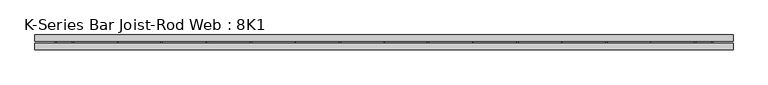
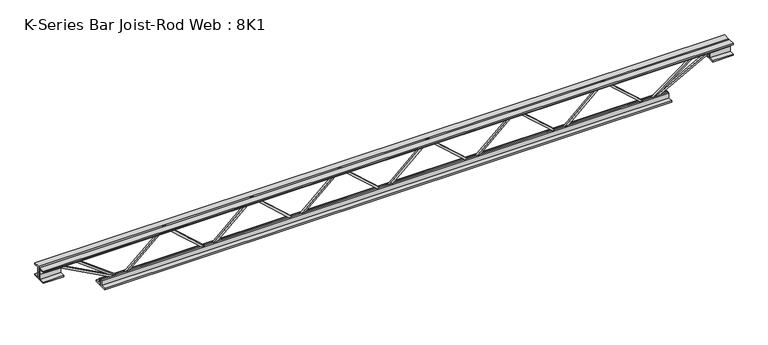
"""IFC4 building model written with IfcOpenShell, lengths in millimetres: beam geometry, K-Series Bar Joist-Rod Web : 8K1."""

from ifc_helpers import new_model, si_unit, frame, origin, place, context, project, spatial, polyline, outline, extrude, source, transform, mapped, element, save


def k_series_bar_joist_rod_web_8k1_279f3ebc(model_context):
    return source(origin(), model_context, "Body", "SweptSolid", [
        extrude(outline(polyline([(-90.4875, 437.278907), (-100.0125, 437.278907), (-100.0125, 442.2774605), (90.4875, 654.566914), (90.4875, 657.269807), (-100.0125, 869.5592605), (-100.0125, 874.557814), (-90.4875, 874.557814), (-90.4875, 873.2063675), (100.0125, 660.916914), (100.0125, 650.919807), (-90.4875, 438.6303535), (-90.4875, 437.278907)])), frame((0.0, -4.7625, 0.0), z_axis=(0.0, 1.0, 0.0), x_axis=(0.0, 0.0, 1.0)), (0.0, 0.0, 1.0), 9.525),
        extrude(outline(polyline([(-90.4875, 0.0), (-100.0125, 0.0), (-100.0125, 4.9985535), (90.4875, 217.288007), (90.4875, 219.9909), (-100.0125, 432.2803535), (-100.0125, 437.278907), (-90.4875, 437.278907), (-90.4875, 435.9274605), (100.0125, 223.638007), (100.0125, 213.6409), (-90.4875, 1.3514465), (-90.4875, 0.0)])), frame((0.0, -4.7625, 0.0), z_axis=(0.0, 1.0, 0.0), x_axis=(0.0, 0.0, 1.0)), (0.0, 0.0, 1.0), 9.525),
        extrude(outline(polyline([(-90.4875, -437.278907), (-100.0125, -437.278907), (-100.0125, -432.2803535), (90.4875, -219.9909), (90.4875, -217.288007), (-100.0125, -4.9985535), (-100.0125, 0.0), (-90.4875, 0.0), (-90.4875, -1.3514465), (100.0125, -213.6409), (100.0125, -223.638007), (-90.4875, -435.9274605), (-90.4875, -437.278907)])), frame((0.0, -4.7625, 0.0), z_axis=(0.0, 1.0, 0.0), x_axis=(0.0, 0.0, 1.0)), (0.0, 0.0, 1.0), 9.525),
        extrude(outline(polyline([(-90.4875, -874.557814), (-100.0125, -874.557814), (-100.0125, -869.5592605), (90.4875, -657.269807), (90.4875, -654.566914), (-100.0125, -442.2774605), (-100.0125, -437.278907), (-90.4875, -437.278907), (-90.4875, -438.6303535), (100.0125, -650.919807), (100.0125, -660.916914), (-90.4875, -873.2063675), (-90.4875, -874.557814)])), frame((0.0, -4.7625, 0.0), z_axis=(0.0, 1.0, 0.0), x_axis=(0.0, 0.0, 1.0)), (0.0, 0.0, 1.0), 9.525),
        extrude(outline(polyline([(-90.4875, 874.557814), (-100.0125, 874.557814), (-100.0125, 879.5563675), (90.4875, 1091.845821), (90.4875, 1094.548714), (-100.0125, 1306.8381675), (-100.0125, 1311.836721), (-90.4875, 1311.836721), (-90.4875, 1310.4852745), (100.0125, 1098.195821), (100.0125, 1088.198714), (-90.4875, 875.9092605), (-90.4875, 874.557814)])), frame((0.0, -4.7625, 0.0), z_axis=(0.0, 1.0, 0.0), x_axis=(0.0, 0.0, 1.0)), (0.0, 0.0, 1.0), 9.525),
        extrude(outline(polyline([(-90.4875, -1311.836721), (-100.0125, -1311.836721), (-100.0125, -1306.8381675), (90.4875, -1094.548714), (90.4875, -1091.845821), (-100.0125, -879.5563675), (-100.0125, -874.557814), (-90.4875, -874.557814), (-90.4875, -875.9092605), (100.0125, -1088.198714), (100.0125, -1098.195821), (-90.4875, -1310.4852745), (-90.4875, -1311.836721)])), frame((0.0, -4.7625, 0.0), z_axis=(0.0, 1.0, 0.0), x_axis=(0.0, 0.0, 1.0)), (0.0, 0.0, 1.0), 9.525),
        extrude(outline(polyline([(4.7625, 101.6), (36.5125, 101.6), (36.5125, 95.25), (11.1125, 95.25), (11.1125, 69.85), (4.7625, 69.85), (4.7625, 101.6)])), frame((-1718.236721, 0.0, 0.0), z_axis=(1.0, 0.0, 0.0), x_axis=(0.0, 1.0, 0.0)), (0.0, 0.0, 1.0), 3436.473442),
        extrude(outline(polyline([(-4.7625, 101.6), (-4.7625, 69.85), (-11.1125, 69.85), (-11.1125, 95.25), (-36.5125, 95.25), (-36.5125, 101.6), (-4.7625, 101.6)])), frame((-1718.236721, 0.0, 0.0), z_axis=(1.0, 0.0, 0.0), x_axis=(0.0, 1.0, 0.0)), (0.0, 0.0, 1.0), 3436.473442),
        extrude(outline(polyline([(-4.7625, 38.1), (-36.5125, 38.1), (-36.5125, 44.45), (-11.1125, 44.45), (-11.1125, 69.85), (-4.7625, 69.85), (-4.7625, 38.1)])), frame((-1718.236721, 0.0, 0.0), z_axis=(1.0, 0.0, 0.0), x_axis=(0.0, 1.0, 0.0)), (0.0, 0.0, 1.0), 101.6),
        extrude(outline(polyline([(36.5125, 38.1), (4.7625, 38.1), (4.7625, 69.85), (11.1125, 69.85), (11.1125, 44.45), (36.5125, 44.45), (36.5125, 38.1)])), frame((-1718.236721, 0.0, 0.0), z_axis=(1.0, 0.0, 0.0), x_axis=(0.0, 1.0, 0.0)), (0.0, 0.0, 1.0), 101.6),
        extrude(outline(polyline([(4.7625, 38.1), (4.7625, 69.85), (11.1125, 69.85), (11.1125, 44.45), (36.5125, 44.45), (36.5125, 38.1), (4.7625, 38.1)])), frame((1616.636721, 0.0, 0.0), z_axis=(1.0, 0.0, 0.0), x_axis=(0.0, 1.0, 0.0)), (0.0, 0.0, 1.0), 101.6),
        extrude(outline(polyline([(-4.7625, 38.1), (-36.5125, 38.1), (-36.5125, 44.45), (-11.1125, 44.45), (-11.1125, 69.85), (-4.7625, 69.85), (-4.7625, 38.1)])), frame((1616.636721, 0.0, 0.0), z_axis=(1.0, 0.0, 0.0), x_axis=(0.0, 1.0, 0.0)), (0.0, 0.0, 1.0), 101.6),
        extrude(outline(polyline([(4.7625, -101.6), (4.7625, -69.85), (11.1125, -69.85), (11.1125, -95.25), (36.5125, -95.25), (36.5125, -101.6), (4.7625, -101.6)])), frame((-1413.436721, 0.0, 0.0), z_axis=(1.0, 0.0, 0.0), x_axis=(0.0, 1.0, 0.0)), (0.0, 0.0, 1.0), 2826.873442),
        extrude(outline(polyline([(-4.7625, -101.6), (-36.5125, -101.6), (-36.5125, -95.25), (-11.1125, -95.25), (-11.1125, -69.85), (-4.7625, -69.85), (-4.7625, -101.6)])), frame((-1413.436721, 0.0, 0.0), z_axis=(1.0, 0.0, 0.0), x_axis=(0.0, 1.0, 0.0)), (0.0, 0.0, 1.0), 2826.873442),
        extrude(outline(polyline([(0.0, -9.525), (0.0, 0.0), (346.6425392, 0.0), (346.6425392, -9.525), (0.0, -9.525)])), frame((-1618.9050195, 4.7625, 65.662372), z_axis=(0.47628314854008014, 0.0, 0.8792919665371384), x_axis=(0.8792919665371384, 0.0, -0.47628314854008014)), (0.0, 0.0, 1.0), 9.525),
        extrude(outline(polyline([(0.0, -9.525), (0.0, 0.0), (273.973029, 0.0), (273.973029, -9.525), (0.0, -9.525)])), frame((-1533.346124, 4.7625, 66.049369), z_axis=(0.6026140623855752, 0.0, 0.7980327636226184), x_axis=(0.7980327636226184, 0.0, -0.6026140623855752)), (0.0, 0.0, 1.0), 9.525),
        extrude(outline(polyline([(0.0, -9.525), (0.0, 0.0), (346.6425392, 0.0), (346.6425392, -9.525), (0.0, -9.525)])), frame((1618.9050195, -4.7625, 65.662372), z_axis=(-0.4762831485400414, 0.0, 0.8792919665371594), x_axis=(-0.8792919665371594, 0.0, -0.4762831485400414)), (0.0, 0.0, 1.0), 9.525),
        extrude(outline(polyline([(0.0, -9.525), (0.0, 0.0), (273.973029, 0.0), (273.973029, -9.525), (0.0, -9.525)])), frame((1533.346124, -4.7625, 66.049369), z_axis=(-0.602614062385554, 0.0, 0.7980327636226345), x_axis=(-0.7980327636226345, 0.0, -0.602614062385554)), (0.0, 0.0, 1.0), 9.525),
    ])


if __name__ == "__main__":
    model = new_model("IFC4")
    model_context = context("Model", 3, world=origin())
    ifc_project = project(units=[si_unit("LENGTHUNIT", "METRE", prefix="MILLI")], contexts=[model_context])
    site = spatial("IfcSite", under=ifc_project)
    building = spatial("IfcBuilding", under=site)
    placement = place(None, origin())
    k_series_bar_joist_rod_web_8k1_shape = k_series_bar_joist_rod_web_8k1_279f3ebc(model_context)
    element("IfcBeam", 1, ObjectType="K-Series Bar Joist-Rod Web : 8K1", at=placement, inside=building, context=model_context, shape_type="MappedRepresentation", body=[
        mapped(k_series_bar_joist_rod_web_8k1_shape, transform((0.0, 0.0, 0.0), x_axis=(1.0, 0.0, 0.0), y_axis=(0.0, 1.0, 0.0), z_axis=(0.0, 0.0, 1.0))),
    ])
    save(model, "model.ifc")

# Revit data of these elements
# Type "K-Series Bar Joist-Rod Web : 8K1"
#   Assembly Code = "B1010350"
#   Wt = 5.1
#   Web Thickness = 0' - 0 3/8"
#   Start Offset [instance default] = 0' - 0"
#   Start Extension [instance default] = 0' - 0"
#   Seat Length = 0' - 4"
#   Seat Depth = 0' - 2 1/2"
#   PanelArrayLength [instance default] = 21' - 4"
#   Panel [instance default] = 1' - 4"
#   End Offset [instance default] = 0' - 0"
#   End Extension [instance default] = 0' - 0"
#   End Panel = 1' - 4"
#   Cord Leg = 0' - 1 1/4"
#   Chord Thickness = 0' - 0 1/4"
#   Length [instance default] = 24' - 0"
#   Depth = 0' - 8"
#   PanelArrayNum [instance default] = 16
#   Rendering Material = none
# Element 1 (IfcBeam, "K-Series Bar Joist-Rod Web : 8K1")
#   PanelArrayLength = 8' - 7.29423"
#   Panel = 1' - 5.21571"
#   PanelArrayNum = 6
